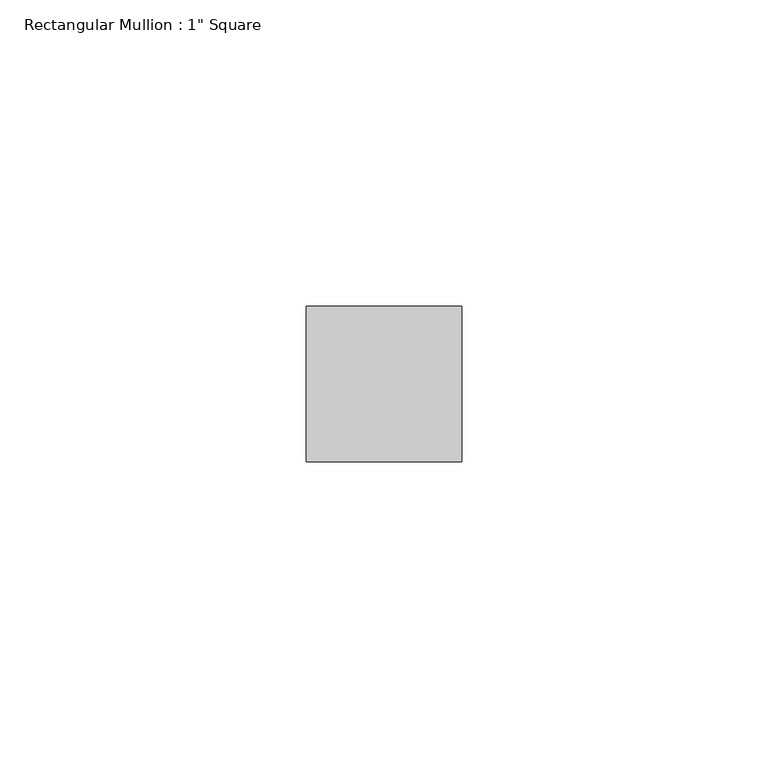
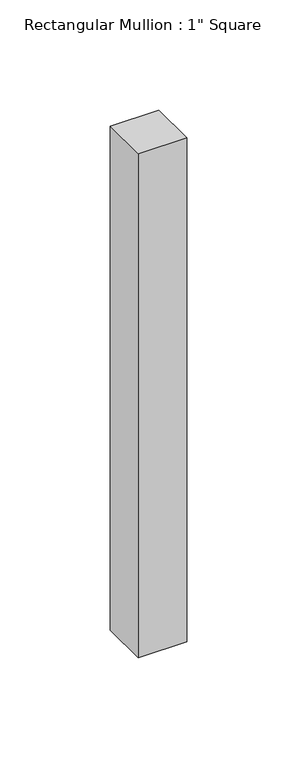
"""IFC4 building model written with IfcOpenShell, lengths in millimetres: member geometry."""

from ifc_helpers import new_model, si_unit, frame, origin, place, context, project, spatial, polyline, outline, extrude, source, transform, mapped, element, save


def member_91e62c05(model_context):
    return source(origin(), model_context, "Body", "SweptSolid", [
        extrude(outline(polyline([(0.0, 12.7), (0.0, -12.7), (-25.4, -12.7), (-25.4, 12.7), (0.0, 12.7)])), frame((0.0, 0.0, -279.4), z_axis=(0.0, 0.0, 1.0), x_axis=(1.0, 0.0, 0.0)), (0.0, 0.0, 1.0), 279.4),
    ])


if __name__ == "__main__":
    model = new_model("IFC4")
    model_context = context("Model", 3, world=origin())
    ifc_project = project(units=[si_unit("LENGTHUNIT", "METRE", prefix="MILLI")], contexts=[model_context])
    site = spatial("IfcSite", under=ifc_project)
    building = spatial("IfcBuilding", under=site)
    placement = place(None, origin())
    member_shape = member_91e62c05(model_context)
    element("IfcMember", 1, ObjectType="Rectangular Mullion : 1\" Square", at=placement, inside=building, context=model_context, shape_type="MappedRepresentation", body=[
        mapped(member_shape, transform((0.0, 0.0, 0.0), x_axis=(1.0, 0.0, 0.0), y_axis=(0.0, 1.0, 0.0), z_axis=(0.0, 0.0, 1.0))),
    ])
    save(model, "model.ifc")

# Revit data of these elements
# Type "Rectangular Mullion : 1\" Square"
#   built-in parameter 1007304 = 0.0833333 (stored number, unit not read)
#   built-in parameter 1007301 = 0.0416667 (stored number, unit not read)
#   built-in parameter 1007300 = 0.0416667 (stored number, unit not read)
# Element 1 (IfcMember, "Rectangular Mullion : 1\" Square")
#   Materials on its faces: "Metal - Aluminum"
# Materials
#   "Metal - Aluminum": class "Metal", colour RGB 247 247 247, transparency 0
